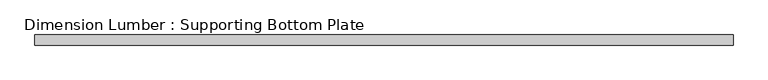
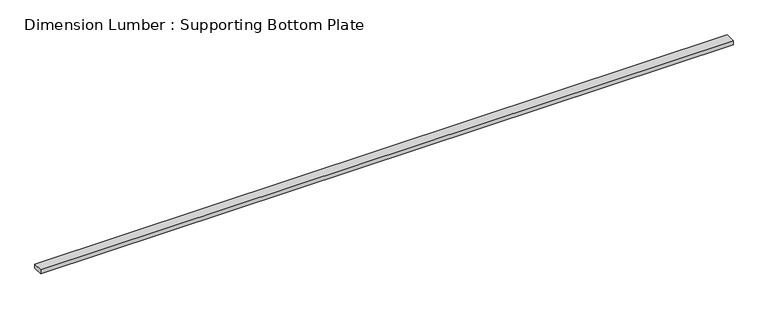
"""IFC4 building model written with IfcOpenShell, lengths in millimetres: beam geometry, Dimension Lumber : Supporting Bottom Plate."""

from ifc_helpers import new_model, si_unit, frame, origin, place, context, project, spatial, polyline, outline, extrude, source, transform, mapped, element, save


def dimension_lumber_supporting_bottom_plate_8d258b52(model_context):
    return source(origin(), model_context, "Body", "SweptSolid", [
        extrude(outline(polyline([(3074.9875, 44.45), (3074.9875, -44.45), (-3074.9875, -44.45), (-3074.9875, 44.45), (3074.9875, 44.45)])), frame((0.0, 0.0, -19.05), z_axis=(0.0, 0.0, 1.0), x_axis=(1.0, 0.0, 0.0)), (0.0, 0.0, 1.0), 38.1),
    ])


if __name__ == "__main__":
    model = new_model("IFC4")
    model_context = context("Model", 3, world=origin())
    ifc_project = project(units=[si_unit("LENGTHUNIT", "METRE", prefix="MILLI")], contexts=[model_context])
    site = spatial("IfcSite", under=ifc_project)
    building = spatial("IfcBuilding", under=site)
    placement = place(None, origin())
    dimension_lumber_supporting_bottom_plate_shape = dimension_lumber_supporting_bottom_plate_8d258b52(model_context)
    element("IfcBeam", 1, ObjectType="Dimension Lumber : Supporting Bottom Plate", at=placement, inside=building, context=model_context, shape_type="MappedRepresentation", body=[
        mapped(dimension_lumber_supporting_bottom_plate_shape, transform((0.0, 0.0, 0.0), x_axis=(1.0, 0.0, 0.0), y_axis=(0.0, 1.0, 0.0), z_axis=(0.0, 0.0, 1.0))),
    ])
    save(model, "model.ifc")

# Revit data of these elements
# Type "Dimension Lumber : Supporting Bottom Plate"
#   Assembly Code = "B10"
#   A = 0.0364583 SF
#   Length [instance default] = 5' - 0"
#   b = 0' - 3 1/2"
#   d = 0' - 1 1/2"
#   Structural Material [instance default] = Softwood, Lumber
# Element 1 (IfcBeam, "Dimension Lumber : Supporting Bottom Plate")
#   Structural Material = Douglas Fir #2
#   Materials on its faces: "Douglas Fir #2"
# Materials
#   "Softwood, Lumber": class "Wood", colour RGB 223 192 134, transparency 0, Description = "Pinus Echinata", Cost = 0
#   "Douglas Fir #2": class "Wood", colour RGB 223 192 134, transparency 0, Description = "Pinus Echinata", Cost = 0
